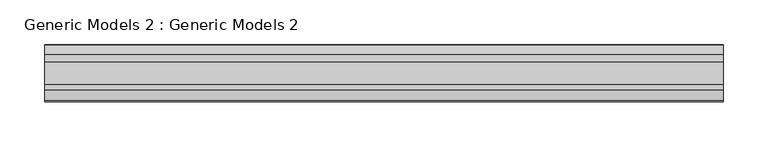
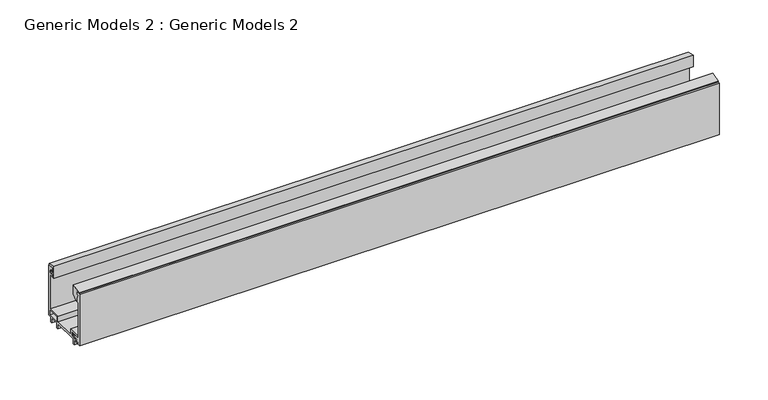
"""IFC4 building model written with IfcOpenShell, lengths in millimetres: proxy geometry, Generic Models 2 : Generic Models 2."""

from ifc_helpers import new_model, si_unit, frame, origin, place, context, project, spatial, polyline, outline, extrude, source, transform, mapped, element, save


def generic_models_2_generic_models_2_43a98067(model_context):
    return source(origin(), model_context, "Body", "SweptSolid", [
        extrude(outline(polyline([(-579078.5739799, 38.4543134), (-579078.5247354, 37.5044445), (-579079.2652904, 37.0107412), (-579080.2786171, 37.6694036), (-579081.6864938, 37.6694036), (-579081.6864938, 35.3570787), (-579084.8288841, 35.3570787), (-579084.8288841, 99.8650152), (-579079.3741689, 99.8650152), (-579079.3741689, 96.7226249), (-579081.1528804, 96.426173), (-579079.3741689, 91.5643616), (-579079.3741689, 87.295454), (-579081.6864938, 87.295454), (-579081.6864938, 42.7683765), (-579069.5319653, 42.7683765), (-579069.5319653, 41.3962277), (-579079.4334593, 39.9817285), (-579079.4334593, 38.9309415), (-579078.5739799, 38.4543134)])), frame((591999.8068336, 0.0, 0.0), z_axis=(1.0, 0.0, 0.0), x_axis=(0.0, 1.0, 0.0)), (0.0, 0.0, 1.0), 755.65),
        extrude(outline(polyline([(-579083.2164454, 101.101348), (-579071.7849999, 104.1497335), (-579071.7849999, 92.5441205), (-579077.8782793, 87.295454), (-579079.0835833, 87.295454), (-579079.0835833, 91.8245902), (-579080.6256201, 96.039491), (-579079.0835833, 96.2964971), (-579079.0835833, 100.0627349), (-579083.2164454, 100.0627349), (-579083.2164454, 101.101348)])), frame((591999.8068336, 0.0, 0.0), z_axis=(1.0, 0.0, 0.0), x_axis=(0.0, 1.0, 0.0)), (0.0, 0.0, 1.0), 755.65),
        extrude(outline(polyline([(-579023.8783705, 88.0069386), (-579028.44373, 88.0069386), (-579028.44373, 90.0525332), (-579027.1393416, 91.3568057), (-579027.1393416, 89.5484886), (-579025.657082, 89.5484886), (-579024.6632617, 91.2698359), (-579024.6632617, 93.551255), (-579025.5486834, 95.450048), (-579027.1393416, 95.450048), (-579027.1393416, 93.4168245), (-579028.44373, 93.639525), (-579028.44373, 98.6792075), (-579021.3288841, 98.0807625), (-579021.3288841, 35.6535306), (-579024.8863071, 35.6535306), (-579024.8863071, 29.36875), (-579026.9021801, 29.36875), (-579026.9021801, 35.6535306), (-579037.8116105, 35.6535306), (-579037.8116105, 29.36875), (-579039.8274835, 29.36875), (-579039.8274835, 35.6535306), (-579070.8956441, 35.6535306), (-579070.8956441, 29.36875), (-579072.9115171, 29.36875), (-579072.9115171, 35.6535306), (-579081.5086227, 35.6535306), (-579081.5086227, 37.0172094), (-579080.6785573, 37.5508228), (-579079.7299112, 36.8986286), (-579072.9115171, 36.8986286), (-579071.6071287, 38.203017), (-579067.8718346, 38.203017), (-579067.8718346, 43.5391515), (-579081.3307515, 43.5391515), (-579081.3307515, 45.0807014), (-579065.8559616, 45.0807014), (-579065.8559616, 38.203017), (-579039.9460643, 38.203017), (-579039.9460643, 45.0807014), (-579023.8783705, 45.0807014), (-579023.8783705, 88.0069386)]), holes=[polyline([(-579024.4712744, 37.7879844), (-579024.4712744, 43.5391515), (-579037.8116105, 43.5391515), (-579037.8116105, 37.7879844), (-579024.4712744, 37.7879844)])]), frame((591999.8068336, 0.0, 0.0), z_axis=(1.0, 0.0, 0.0), x_axis=(0.0, 1.0, 0.0)), (0.0, 0.0, 1.0), 755.65),
        extrude(outline(polyline([(-579031.7849999, 102.6595575), (-579021.8263604, 100.4407933), (-579021.8263604, 98.3393783), (-579028.7505755, 98.9217889), (-579028.7505755, 93.4814891), (-579026.8269234, 93.1530607), (-579026.8269234, 95.1913241), (-579025.8025744, 95.1913241), (-579024.9625289, 93.3898405), (-579024.9625289, 91.309542), (-579025.8229772, 89.8192017), (-579026.9121641, 89.8192017), (-579026.9121641, 92.0735899), (-579028.7505755, 90.2351786), (-579028.7505755, 88.0069386), (-579031.7849999, 88.0069386), (-579031.7849999, 102.6595575)])), frame((591999.8068336, 0.0, 0.0), z_axis=(1.0, 0.0, 0.0), x_axis=(0.0, 1.0, 0.0)), (0.0, 0.0, 1.0), 755.65),
    ])


if __name__ == "__main__":
    model = new_model("IFC4")
    model_context = context("Model", 3, world=origin())
    ifc_project = project(units=[si_unit("LENGTHUNIT", "METRE", prefix="MILLI")], contexts=[model_context])
    site = spatial("IfcSite", under=ifc_project)
    building = spatial("IfcBuilding", under=site)
    placement = place(None, origin())
    generic_models_2_generic_models_2_shape = generic_models_2_generic_models_2_43a98067(model_context)
    element("IfcBuildingElementProxy", 1, Name="Generic Models 2 : Generic Models 2", ObjectType="Generic Models 2 : Generic Models 2", at=placement, inside=building, context=model_context, shape_type="MappedRepresentation", body=[
        mapped(generic_models_2_generic_models_2_shape, transform((0.0, 0.0, 0.0), x_axis=(1.0, 0.0, 0.0), y_axis=(0.0, 1.0, 0.0), z_axis=(0.0, 0.0, 1.0))),
    ])
    save(model, "model.ifc")

# Revit data of these elements
# Element 1 (IfcBuildingElementProxy, "Generic Models 2 : Generic Models 2")
#   Materials on its faces: "THERMAL BROKEN ALUMINUM STOREFRONT FOR POLYCARBONATE"
# Materials
#   "THERMAL BROKEN ALUMINUM STOREFRONT FOR POLYCARBONATE": class "Unassigned", colour RGB 244 244 244, transparency 0, Keynote = "M07611300.01", Cost = 0
